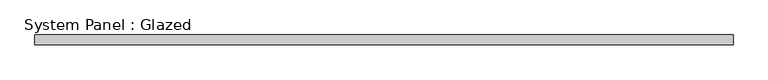
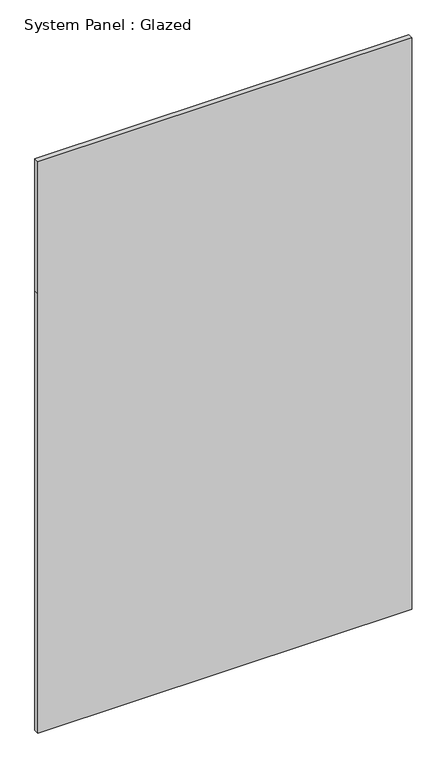
"""IFC4 building model written with IfcOpenShell, lengths in millimetres: plate geometry, System Panel : Glazed."""

import ifcopenshell
import ifcopenshell.guid

model = None  # the IFC model being written
_history = None  # IfcOwnerHistory: only IFC2X3 demands one
_inside = {}  # id of a spatial element -> (the spatial element, [elements in it])
_under = {}  # id of a project, library or spatial element -> (it, [spatial elements below it])
_declared = {}  # id of a project -> (the project, [libraries it declares])
_typed = {}  # id of a type object -> (the type object, [elements of that type])
_made_of = {}  # id of a material, layer set ... -> (it, [elements and type objects made of it])


def new_model(schema):
    """Start an empty IFC model of exactly this schema.

    Asked for "IFC4X3", IfcOpenShell would pick the latest addendum, in which some entities
    have other attributes; the version numbers below select the first issue.
    IFC2X3 requires an IfcOwnerHistory on every rooted entity: one is made here for all.
    """
    global model, _history
    if schema == "IFC4X3":
        model = ifcopenshell.file(schema_version=(4, 3, 0, 0))
    else:
        model = ifcopenshell.file(schema=schema)
    _inside.clear()
    _under.clear()
    _declared.clear()
    _typed.clear()
    _made_of.clear()
    _history = None
    if model.schema == "IFC2X3":
        org = make("IfcOrganization", Name="unknown")
        user = make(
            "IfcPersonAndOrganization",
            ThePerson=make("IfcPerson", FamilyName="unknown"),
            TheOrganization=org,
        )
        app = make(
            "IfcApplication",
            ApplicationDeveloper=org,
            Version="unknown",
            ApplicationFullName="unknown",
            ApplicationIdentifier="unknown",
        )
        _history = make(
            "IfcOwnerHistory",
            OwningUser=user,
            OwningApplication=app,
            ChangeAction="ADDED",
            CreationDate=0,
        )
    return model


def make(cls, **values):
    """One entity of the class cls with the attributes given. An attribute that is None is left unset."""
    return model.create_entity(
        cls, **{name: value for name, value in values.items() if value is not None}
    )


def rooted(cls, **values):
    """An entity with a GlobalId (a new one), such as an element, a storey or a relation."""
    return make(cls, GlobalId=ifcopenshell.guid.new(), OwnerHistory=_history, **values)


def si_unit(unit_type, name, prefix=None):
    """IfcSIUnit, for example si_unit("LENGTHUNIT", "METRE", prefix="MILLI")."""
    return make("IfcSIUnit", UnitType=unit_type, Prefix=prefix, Name=name)


def assignment(units):
    """IfcUnitAssignment: the units of a project."""
    return None if units is None else make("IfcUnitAssignment", Units=units)


def point(xyz):
    """IfcCartesianPoint."""
    return None if xyz is None else make("IfcCartesianPoint", Coordinates=xyz)


def direction(xyz):
    """IfcDirection."""
    return None if xyz is None else make("IfcDirection", DirectionRatios=xyz)


def frame(location, z_axis=None, x_axis=None):
    """IfcAxis2Placement3D, a coordinate frame: its origin and axes. An axis left out is left unset."""
    return make(
        "IfcAxis2Placement3D",
        Location=point(location),
        Axis=direction(z_axis),
        RefDirection=direction(x_axis),
    )


def origin():
    """The frame at (0, 0, 0) with its axes left unset."""
    return frame((0.0, 0.0, 0.0))


def place(relative_to, where):
    """IfcLocalPlacement: puts the frame where relative to a parent placement (None: the world)."""
    return make(
        "IfcLocalPlacement", PlacementRelTo=relative_to, RelativePlacement=where
    )


def context(
    kind, dimensions, precision=None, world=None, true_north=None, identifier=None
):
    """IfcGeometricRepresentationContext, for example the 3D "Model" context."""
    return make(
        "IfcGeometricRepresentationContext",
        ContextIdentifier=identifier,
        ContextType=kind,
        CoordinateSpaceDimension=dimensions,
        Precision=precision,
        WorldCoordinateSystem=world,
        TrueNorth=true_north,
    )


def project(units=None, contexts=None):
    """IfcProject with its units and contexts."""
    return rooted(
        "IfcProject",
        Name="project",
        RepresentationContexts=contexts,
        UnitsInContext=assignment(units),
    )


def spatial(cls, under=None, at=None, **own):
    """A site, building, storey or space (cls), placed at a placement, below another one or the project."""
    s = rooted(cls, ObjectPlacement=at, **own)
    if under is not None:
        _under.setdefault(under.id(), (under, []))[1].append(s)
    return s


def polyline(points):
    """IfcPolyline through the points."""
    return make("IfcPolyline", Points=[point(p) for p in points])


def outline(outer, holes=None, kind="AREA"):
    """IfcArbitraryClosedProfileDef: a profile drawn as a closed curve; with holes, ...WithVoids."""
    if holes is None:
        return make("IfcArbitraryClosedProfileDef", ProfileType=kind, OuterCurve=outer)
    return make(
        "IfcArbitraryProfileDefWithVoids",
        ProfileType=kind,
        OuterCurve=outer,
        InnerCurves=holes,
    )


def extrude(swept, where, along, depth):
    """IfcExtrudedAreaSolid: the profile swept, set in the frame where, extruded along a direction by depth."""
    return make(
        "IfcExtrudedAreaSolid",
        SweptArea=swept,
        Position=where,
        ExtrudedDirection=direction(along),
        Depth=depth,
    )


def shape(context_of_items, identifier, shape_type, items):
    """IfcShapeRepresentation: the items that make up one representation, for example the "Body"."""
    return make(
        "IfcShapeRepresentation",
        ContextOfItems=context_of_items,
        RepresentationIdentifier=identifier,
        RepresentationType=shape_type,
        Items=items,
    )


def source(mapping_origin, context_of_items, identifier, shape_type, items):
    """IfcRepresentationMap: a shape defined once, which mapped items show again and again."""
    return make(
        "IfcRepresentationMap",
        MappingOrigin=mapping_origin,
        MappedRepresentation=shape(context_of_items, identifier, shape_type, items),
    )


def transform(
    local_origin,
    x_axis=None,
    y_axis=None,
    z_axis=None,
    scale=None,
    scale2=None,
    scale3=None,
    uniform=True,
):
    """IfcCartesianTransformationOperator3D, or its non-uniform kind. x_axis, y_axis, z_axis: its Axis1, 2, 3."""
    if uniform:
        return make(
            "IfcCartesianTransformationOperator3D",
            Axis1=direction(x_axis),
            Axis2=direction(y_axis),
            LocalOrigin=point(local_origin),
            Scale=scale,
            Axis3=direction(z_axis),
        )
    return make(
        "IfcCartesianTransformationOperator3DnonUniform",
        Axis1=direction(x_axis),
        Axis2=direction(y_axis),
        LocalOrigin=point(local_origin),
        Scale=scale,
        Axis3=direction(z_axis),
        Scale2=scale2,
        Scale3=scale3,
    )


def mapped(mapping_source, mapping_target):
    """IfcMappedItem: shows the shape of a source again, moved by a transform."""
    return make(
        "IfcMappedItem", MappingSource=mapping_source, MappingTarget=mapping_target
    )


def made_of(thing, what):
    """Note that an element or type object is made of a material, layer set ...; save() writes the relation."""
    if what is not None:
        _made_of.setdefault(what.id(), (what, []))[1].append(thing)
    return thing


def element(
    cls,
    number,
    at=None,
    inside=None,
    cuts=None,
    type_object=None,
    material=None,
    context=None,
    identifier="Body",
    shape_type=None,
    held_by="IfcProductDefinitionShape",
    body=None,
    shapes=None,
    **own,
):
    """One element of the class cls, such as IfcWall. Its Tag is "e" and its number.

    at: its placement. inside: the storey or other place that contains it. cuts: it is an
    opening in that element (IfcRelVoidsElement). A single representation is given by context,
    identifier, shape_type and body (its items); several are given by shapes. held_by: the class
    of the entity that holds the representations. save() writes the other relations.
    """
    e = rooted(cls, Tag="e%d" % number, ObjectPlacement=at, **own)
    if body is not None:
        shapes = [shape(context, identifier, shape_type, body)]
    if shapes is not None:
        e.Representation = make(held_by, Representations=shapes)
    if inside is not None:
        _inside.setdefault(inside.id(), (inside, []))[1].append(e)
    if cuts is not None:
        rooted(
            "IfcRelVoidsElement", RelatingBuildingElement=cuts, RelatedOpeningElement=e
        )
    if type_object is not None:
        _typed.setdefault(type_object.id(), (type_object, []))[1].append(e)
    return made_of(e, material)


def aggregate(whole, parts):
    """IfcRelAggregates: a whole, such as a stair, and the parts it consists of."""
    return rooted("IfcRelAggregates", RelatingObject=whole, RelatedObjects=parts)


def save(model, path):
    """Write the relations noted so far, then the file.

    IfcRelAggregates (storeys below a building ...), IfcRelContainedInSpatialStructure (elements
    in a storey), IfcRelDefinesByType, IfcRelAssociatesMaterial and IfcRelDeclares: one each for
    every whole, place, type object, material and project.
    """
    for whole, parts in _under.values():
        aggregate(whole, parts)
    for where, things in _inside.values():
        rooted(
            "IfcRelContainedInSpatialStructure",
            RelatedElements=things,
            RelatingStructure=where,
        )
    for kind, things in _typed.values():
        rooted("IfcRelDefinesByType", RelatedObjects=things, RelatingType=kind)
    for what, things in _made_of.values():
        rooted("IfcRelAssociatesMaterial", RelatedObjects=things, RelatingMaterial=what)
    for by, libraries in _declared.values():
        rooted("IfcRelDeclares", RelatingContext=by, RelatedDefinitions=libraries)
    model.write(path)


def system_panel_glazed_640a10fc(model_context):
    return source(origin(), model_context, "Body", "SweptSolid", [
        extrude(outline(polyline([(0.0, -905.5833335), (0.0, 905.5833335), (2250.0, 905.5833335), (2925.0, 905.5833335), (2925.0, -905.5833335), (2250.0, -905.5833335), (0.0, -905.5833335)])), frame((0.0, 24.5, 0.0), z_axis=(0.0, 1.0, 0.0), x_axis=(0.0, 0.0, 1.0)), (0.0, 0.0, 1.0), 25.0),
    ])


if __name__ == "__main__":
    model = new_model("IFC4")
    model_context = context("Model", 3, world=origin())
    ifc_project = project(units=[si_unit("LENGTHUNIT", "METRE", prefix="MILLI")], contexts=[model_context])
    site = spatial("IfcSite", under=ifc_project)
    building = spatial("IfcBuilding", under=site)
    placement = place(None, origin())
    system_panel_glazed_shape = system_panel_glazed_640a10fc(model_context)
    element("IfcPlate", 1, ObjectType="System Panel : Glazed", at=placement, inside=building, context=model_context, shape_type="MappedRepresentation", body=[
        mapped(system_panel_glazed_shape, transform((0.0, 0.0, 0.0), x_axis=(1.0, 0.0, 0.0), y_axis=(0.0, 1.0, 0.0), z_axis=(0.0, 0.0, 1.0))),
    ])
    save(model, "model.ifc")

# Revit data of these elements
# Element 1 (IfcPlate, "System Panel : Glazed")
#   Materials on its faces: "Glass"
# Materials
#   "Glass": class "Glass", colour RGB 0 128 192, transparency 0.9
